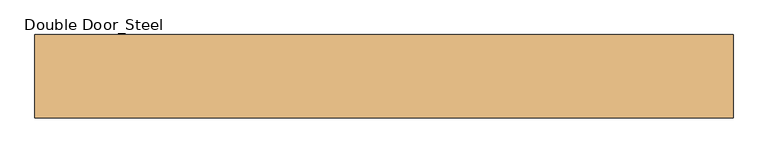
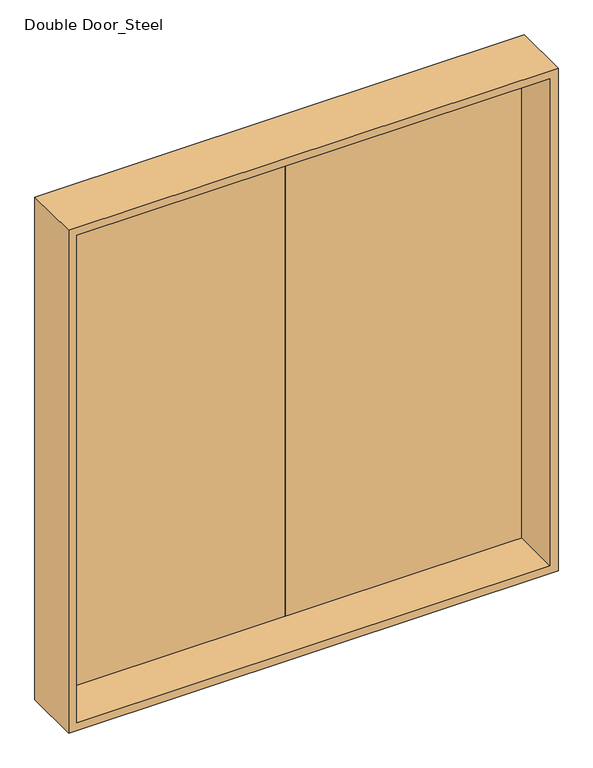
"""IFC4 building model written with IfcOpenShell, lengths in millimetres: door geometry, Double Door_Steel : H_DR_AR_B12_Double Door_Sliding_W2100xH2280_SD3."""

import ifcopenshell
import ifcopenshell.guid

model = None  # the IFC model being written
_history = None  # IfcOwnerHistory: only IFC2X3 demands one
_inside = {}  # id of a spatial element -> (the spatial element, [elements in it])
_under = {}  # id of a project, library or spatial element -> (it, [spatial elements below it])
_declared = {}  # id of a project -> (the project, [libraries it declares])
_typed = {}  # id of a type object -> (the type object, [elements of that type])
_made_of = {}  # id of a material, layer set ... -> (it, [elements and type objects made of it])


def new_model(schema):
    """Start an empty IFC model of exactly this schema.

    Asked for "IFC4X3", IfcOpenShell would pick the latest addendum, in which some entities
    have other attributes; the version numbers below select the first issue.
    IFC2X3 requires an IfcOwnerHistory on every rooted entity: one is made here for all.
    """
    global model, _history
    if schema == "IFC4X3":
        model = ifcopenshell.file(schema_version=(4, 3, 0, 0))
    else:
        model = ifcopenshell.file(schema=schema)
    _inside.clear()
    _under.clear()
    _declared.clear()
    _typed.clear()
    _made_of.clear()
    _history = None
    if model.schema == "IFC2X3":
        org = make("IfcOrganization", Name="unknown")
        user = make(
            "IfcPersonAndOrganization",
            ThePerson=make("IfcPerson", FamilyName="unknown"),
            TheOrganization=org,
        )
        app = make(
            "IfcApplication",
            ApplicationDeveloper=org,
            Version="unknown",
            ApplicationFullName="unknown",
            ApplicationIdentifier="unknown",
        )
        _history = make(
            "IfcOwnerHistory",
            OwningUser=user,
            OwningApplication=app,
            ChangeAction="ADDED",
            CreationDate=0,
        )
    return model


def make(cls, **values):
    """One entity of the class cls with the attributes given. An attribute that is None is left unset."""
    return model.create_entity(
        cls, **{name: value for name, value in values.items() if value is not None}
    )


def rooted(cls, **values):
    """An entity with a GlobalId (a new one), such as an element, a storey or a relation."""
    return make(cls, GlobalId=ifcopenshell.guid.new(), OwnerHistory=_history, **values)


def si_unit(unit_type, name, prefix=None):
    """IfcSIUnit, for example si_unit("LENGTHUNIT", "METRE", prefix="MILLI")."""
    return make("IfcSIUnit", UnitType=unit_type, Prefix=prefix, Name=name)


def assignment(units):
    """IfcUnitAssignment: the units of a project."""
    return None if units is None else make("IfcUnitAssignment", Units=units)


def point(xyz):
    """IfcCartesianPoint."""
    return None if xyz is None else make("IfcCartesianPoint", Coordinates=xyz)


def direction(xyz):
    """IfcDirection."""
    return None if xyz is None else make("IfcDirection", DirectionRatios=xyz)


def frame(location, z_axis=None, x_axis=None):
    """IfcAxis2Placement3D, a coordinate frame: its origin and axes. An axis left out is left unset."""
    return make(
        "IfcAxis2Placement3D",
        Location=point(location),
        Axis=direction(z_axis),
        RefDirection=direction(x_axis),
    )


def origin():
    """The frame at (0, 0, 0) with its axes left unset."""
    return frame((0.0, 0.0, 0.0))


def place(relative_to, where):
    """IfcLocalPlacement: puts the frame where relative to a parent placement (None: the world)."""
    return make(
        "IfcLocalPlacement", PlacementRelTo=relative_to, RelativePlacement=where
    )


def context(
    kind, dimensions, precision=None, world=None, true_north=None, identifier=None
):
    """IfcGeometricRepresentationContext, for example the 3D "Model" context."""
    return make(
        "IfcGeometricRepresentationContext",
        ContextIdentifier=identifier,
        ContextType=kind,
        CoordinateSpaceDimension=dimensions,
        Precision=precision,
        WorldCoordinateSystem=world,
        TrueNorth=true_north,
    )


def project(units=None, contexts=None):
    """IfcProject with its units and contexts."""
    return rooted(
        "IfcProject",
        Name="project",
        RepresentationContexts=contexts,
        UnitsInContext=assignment(units),
    )


def spatial(cls, under=None, at=None, **own):
    """A site, building, storey or space (cls), placed at a placement, below another one or the project."""
    s = rooted(cls, ObjectPlacement=at, **own)
    if under is not None:
        _under.setdefault(under.id(), (under, []))[1].append(s)
    return s


def polyline(points):
    """IfcPolyline through the points."""
    return make("IfcPolyline", Points=[point(p) for p in points])


def outline(outer, holes=None, kind="AREA"):
    """IfcArbitraryClosedProfileDef: a profile drawn as a closed curve; with holes, ...WithVoids."""
    if holes is None:
        return make("IfcArbitraryClosedProfileDef", ProfileType=kind, OuterCurve=outer)
    return make(
        "IfcArbitraryProfileDefWithVoids",
        ProfileType=kind,
        OuterCurve=outer,
        InnerCurves=holes,
    )


def extrude(swept, where, along, depth):
    """IfcExtrudedAreaSolid: the profile swept, set in the frame where, extruded along a direction by depth."""
    return make(
        "IfcExtrudedAreaSolid",
        SweptArea=swept,
        Position=where,
        ExtrudedDirection=direction(along),
        Depth=depth,
    )


def faces_of(points, faces, orient=None, outer=None):
    """IfcFace entities. A face is a list of loops; a loop is a list of indices into points, from 0.

    orient and outer hold one flag for each loop. By default every Orientation is true, the
    first loop of a face is its IfcFaceOuterBound and the others are IfcFaceBound.
    """
    made = []
    for i, loops in enumerate(faces):
        bounds = []
        for j, loop in enumerate(loops):
            is_outer = j == 0 if outer is None else outer[i][j]
            bounds.append(
                make(
                    "IfcFaceOuterBound" if is_outer else "IfcFaceBound",
                    Bound=make("IfcPolyLoop", Polygon=[points[k] for k in loop]),
                    Orientation=True if orient is None else orient[i][j],
                )
            )
        made.append(make("IfcFace", Bounds=bounds))
    return made


def faceted_brep(points, faces, orient=None, outer=None, voids=None):
    """IfcFacetedBrep: a solid bounded by flat faces; with voids (closed shells), ...WithVoids."""
    shared = [point(p) for p in points]
    hull = make("IfcClosedShell", CfsFaces=faces_of(shared, faces, orient, outer))
    if voids is None:
        return make("IfcFacetedBrep", Outer=hull)
    return make(
        "IfcFacetedBrepWithVoids",
        Outer=hull,
        Voids=[
            make(cls, CfsFaces=faces_of(shared, fs, o, b)) for cls, fs, o, b in voids
        ],
    )


def shape(context_of_items, identifier, shape_type, items):
    """IfcShapeRepresentation: the items that make up one representation, for example the "Body"."""
    return make(
        "IfcShapeRepresentation",
        ContextOfItems=context_of_items,
        RepresentationIdentifier=identifier,
        RepresentationType=shape_type,
        Items=items,
    )


def source(mapping_origin, context_of_items, identifier, shape_type, items):
    """IfcRepresentationMap: a shape defined once, which mapped items show again and again."""
    return make(
        "IfcRepresentationMap",
        MappingOrigin=mapping_origin,
        MappedRepresentation=shape(context_of_items, identifier, shape_type, items),
    )


def transform(
    local_origin,
    x_axis=None,
    y_axis=None,
    z_axis=None,
    scale=None,
    scale2=None,
    scale3=None,
    uniform=True,
):
    """IfcCartesianTransformationOperator3D, or its non-uniform kind. x_axis, y_axis, z_axis: its Axis1, 2, 3."""
    if uniform:
        return make(
            "IfcCartesianTransformationOperator3D",
            Axis1=direction(x_axis),
            Axis2=direction(y_axis),
            LocalOrigin=point(local_origin),
            Scale=scale,
            Axis3=direction(z_axis),
        )
    return make(
        "IfcCartesianTransformationOperator3DnonUniform",
        Axis1=direction(x_axis),
        Axis2=direction(y_axis),
        LocalOrigin=point(local_origin),
        Scale=scale,
        Axis3=direction(z_axis),
        Scale2=scale2,
        Scale3=scale3,
    )


def mapped(mapping_source, mapping_target):
    """IfcMappedItem: shows the shape of a source again, moved by a transform."""
    return make(
        "IfcMappedItem", MappingSource=mapping_source, MappingTarget=mapping_target
    )


def made_of(thing, what):
    """Note that an element or type object is made of a material, layer set ...; save() writes the relation."""
    if what is not None:
        _made_of.setdefault(what.id(), (what, []))[1].append(thing)
    return thing


def element(
    cls,
    number,
    at=None,
    inside=None,
    cuts=None,
    type_object=None,
    material=None,
    context=None,
    identifier="Body",
    shape_type=None,
    held_by="IfcProductDefinitionShape",
    body=None,
    shapes=None,
    **own,
):
    """One element of the class cls, such as IfcWall. Its Tag is "e" and its number.

    at: its placement. inside: the storey or other place that contains it. cuts: it is an
    opening in that element (IfcRelVoidsElement). A single representation is given by context,
    identifier, shape_type and body (its items); several are given by shapes. held_by: the class
    of the entity that holds the representations. save() writes the other relations.
    """
    e = rooted(cls, Tag="e%d" % number, ObjectPlacement=at, **own)
    if body is not None:
        shapes = [shape(context, identifier, shape_type, body)]
    if shapes is not None:
        e.Representation = make(held_by, Representations=shapes)
    if inside is not None:
        _inside.setdefault(inside.id(), (inside, []))[1].append(e)
    if cuts is not None:
        rooted(
            "IfcRelVoidsElement", RelatingBuildingElement=cuts, RelatedOpeningElement=e
        )
    if type_object is not None:
        _typed.setdefault(type_object.id(), (type_object, []))[1].append(e)
    return made_of(e, material)


def aggregate(whole, parts):
    """IfcRelAggregates: a whole, such as a stair, and the parts it consists of."""
    return rooted("IfcRelAggregates", RelatingObject=whole, RelatedObjects=parts)


def save(model, path):
    """Write the relations noted so far, then the file.

    IfcRelAggregates (storeys below a building ...), IfcRelContainedInSpatialStructure (elements
    in a storey), IfcRelDefinesByType, IfcRelAssociatesMaterial and IfcRelDeclares: one each for
    every whole, place, type object, material and project.
    """
    for whole, parts in _under.values():
        aggregate(whole, parts)
    for where, things in _inside.values():
        rooted(
            "IfcRelContainedInSpatialStructure",
            RelatedElements=things,
            RelatingStructure=where,
        )
    for kind, things in _typed.values():
        rooted("IfcRelDefinesByType", RelatedObjects=things, RelatingType=kind)
    for what, things in _made_of.values():
        rooted("IfcRelAssociatesMaterial", RelatedObjects=things, RelatingMaterial=what)
    for by, libraries in _declared.values():
        rooted("IfcRelDeclares", RelatingContext=by, RelatedDefinitions=libraries)
    model.write(path)


def double_door_steel_0cd5a1b8(model_context):
    return source(origin(), model_context, "Body", "SolidModel", [
        extrude(outline(polyline([(1030.0, 85.0), (0.0, 85.0), (0.0, 125.0), (1030.0, 125.0), (1030.0, 85.0)])), frame((0.0, 0.0, 20.0), z_axis=(0.0, 0.0, 1.0), x_axis=(1.0, 0.0, 0.0)), (0.0, 0.0, 1.0), 2240.0),
        extrude(outline(polyline([(0.0, 85.0), (-1030.0, 85.0), (-1030.0, 125.0), (0.0, 125.0), (0.0, 85.0)])), frame((0.0, 0.0, 20.0), z_axis=(0.0, 0.0, 1.0), x_axis=(1.0, 0.0, 0.0)), (0.0, 0.0, 1.0), 2240.0),
        faceted_brep([(1050.0, -125.0, 2280.0), (1050.0, 125.0, 2280.0), (-1050.0, 125.0, 2280.0), (-1050.0, -125.0, 2280.0), (1015.0, 85.0, 2245.0), (1015.0, -125.0, 2245.0), (-1015.0, -125.0, 2245.0), (-1015.0, 85.0, 2245.0), (1030.0, 125.0, 2260.0), (1030.0, 85.0, 2260.0), (-1030.0, 85.0, 2260.0), (-1030.0, 125.0, 2260.0), (-1050.0, 125.0, 0.0), (-1050.0, -125.0, 0.0), (-1015.0, -125.0, 35.0), (-1015.0, 85.0, 35.0), (-1030.0, 85.0, 20.0), (-1030.0, 125.0, 20.0), (1050.0, 125.0, 0.0), (1030.0, 125.0, 20.0), (1050.0, -125.0, 0.0), (1015.0, -125.0, 35.0), (1015.0, 85.0, 35.0), (1030.0, 85.0, 20.0)], [[[0, 1, 2, 3]], [[4, 5, 6, 7]], [[8, 9, 10, 11]], [[3, 2, 12, 13]], [[7, 6, 14, 15]], [[11, 10, 16, 17]], [[18, 12, 2, 1], [8, 11, 17, 19]], [[13, 12, 18, 20]], [[0, 3, 13, 20], [21, 14, 6, 5]], [[15, 14, 21, 22]], [[23, 16, 10, 9], [4, 7, 15, 22]], [[17, 16, 23, 19]], [[20, 18, 1, 0]], [[22, 21, 5, 4]], [[19, 23, 9, 8]]]),
    ])


if __name__ == "__main__":
    model = new_model("IFC4")
    model_context = context("Model", 3, world=origin())
    ifc_project = project(units=[si_unit("LENGTHUNIT", "METRE", prefix="MILLI")], contexts=[model_context])
    site = spatial("IfcSite", under=ifc_project)
    building = spatial("IfcBuilding", under=site)
    placement = place(None, origin())
    double_door_steel_shape = double_door_steel_0cd5a1b8(model_context)
    element("IfcDoor", 1, ObjectType="Double Door_Steel : H_DR_AR_B12_Double Door_Sliding_W2100xH2280_SD3", at=placement, inside=building, context=model_context, shape_type="MappedRepresentation", body=[
        mapped(double_door_steel_shape, transform((0.0, 0.0, 0.0), x_axis=(1.0, 0.0, 0.0), y_axis=(0.0, 1.0, 0.0), z_axis=(0.0, 0.0, 1.0))),
    ])
    save(model, "model.ifc")

# Revit data of these elements
# Type "Double Door_Steel : H_DR_AR_B12_Double Door_Sliding_W2100xH2280_SD3"
#   Type Mark = "445"
#   프레임 = ""
#   철물 = ""
#   유리/마감 = ""
#   위치/개소 = ""
#   부호 = "1/SD"
#   문번호 = "3"
#   문기호 = "SD"
#   Analytic Construction = "<None>"
#   Height = 2280 mm
#   Width = 2100 mm
#   Define Thermal Properties by = 1
#   문 틀 = none
#   문 = none
#   Function = (empty or 0)
#   Assembly Code = ""
#   Wall Closure = (empty or 0)
